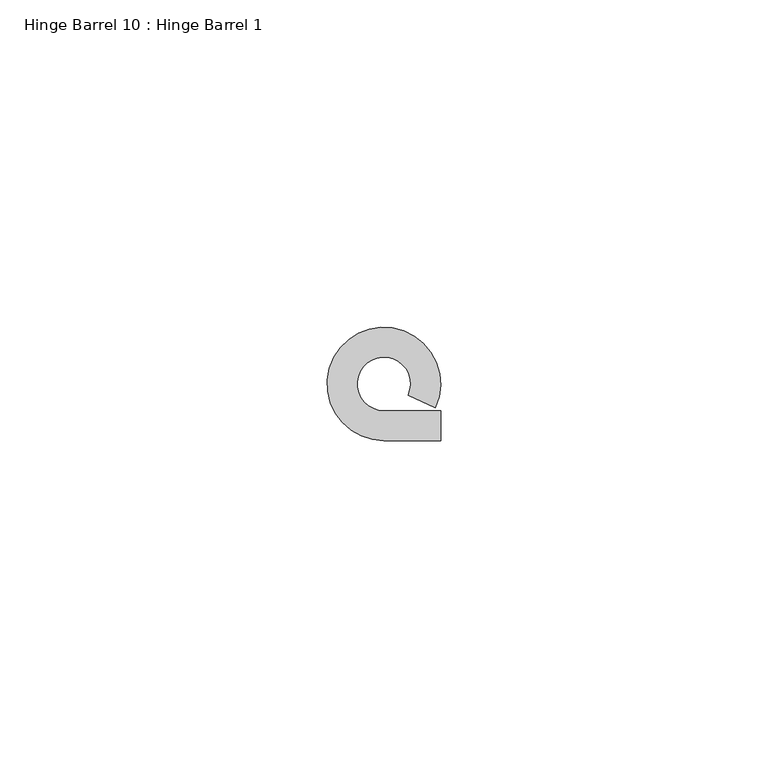
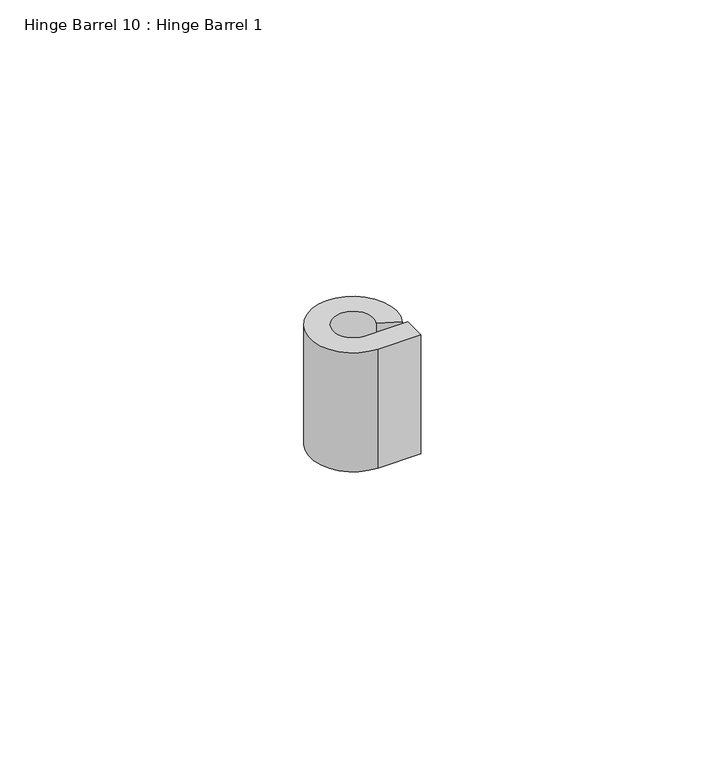
"""IFC4 building model written with IfcOpenShell, lengths in millimetres: proxy geometry, Hinge Barrel 10 : Hinge Barrel 1."""

from ifc_helpers import new_model, si_unit, point, frame, frame_2d, origin, place, context, project, spatial, polyline, circle_curve, trimmed, segment, composite_curve, outline, extrude, source, transform, mapped, element, save


def hinge_barrel_10_hinge_barrel_1_181395a2(model_context):
    return source(origin(), model_context, "Body", "SweptSolid", [
        extrude(outline(composite_curve([segment(polyline([(587323.2214739, -531780.6943841), (587327.7934739, -531780.6943841), (587327.7934739, -531785.2584466), (587319.1320739, -531785.2584466)]), True, "CONTINUOUS"), segment(trimmed(circle_curve(frame_2d((587319.1320739, -531776.6049841)), 8.6534625), [point((587319.1320739, -531785.2584466))], [point((587326.986084, -531780.2377433))], False, "CARTESIAN"), True, "CONTINUOUS"), segment(polyline([(587326.986084, -531780.2377433), (587322.8436736, -531778.321731)]), True, "CONTINUOUS"), segment(trimmed(circle_curve(frame_2d((587319.1320739, -531776.6049841)), 4.0894), [point((587322.8436736, -531778.321731))], [point((587319.1320739, -531780.6943841))], True, "CARTESIAN"), True, "CONTINUOUS"), segment(polyline([(587319.1320739, -531780.6943841), (587323.2214739, -531780.6943841)]), True, "CONTINUOUS")], self_intersect=False)), frame((0.0, 0.0, 2038.35), z_axis=(0.0, 0.0, 1.0), x_axis=(1.0, 0.0, 0.0)), (0.0, 0.0, 1.0), 25.4),
    ])


if __name__ == "__main__":
    model = new_model("IFC4")
    model_context = context("Model", 3, world=origin())
    ifc_project = project(units=[si_unit("LENGTHUNIT", "METRE", prefix="MILLI")], contexts=[model_context])
    site = spatial("IfcSite", under=ifc_project)
    building = spatial("IfcBuilding", under=site)
    placement = place(None, origin())
    hinge_barrel_10_hinge_barrel_1_shape = hinge_barrel_10_hinge_barrel_1_181395a2(model_context)
    element("IfcBuildingElementProxy", 1, Name="Hinge Barrel 10 : Hinge Barrel 1", ObjectType="Hinge Barrel 10 : Hinge Barrel 1", at=placement, inside=building, context=model_context, shape_type="MappedRepresentation", body=[
        mapped(hinge_barrel_10_hinge_barrel_1_shape, transform((0.0, 0.0, 0.0), x_axis=(1.0, 0.0, 0.0), y_axis=(0.0, 1.0, 0.0), z_axis=(0.0, 0.0, 1.0))),
    ])
    save(model, "model.ifc")

# Revit data of these elements
# Element 1 (IfcBuildingElementProxy, "Hinge Barrel 10 : Hinge Barrel 1")
#   Materials on its faces: "6\"X6\" WELD-ON STL BUTT HINGE"
# Materials
#   "6\"X6\" WELD-ON STL BUTT HINGE": class "Metal", colour RGB 189 187 185, transparency 0, Description = "Carbon steel", Cost = 0
